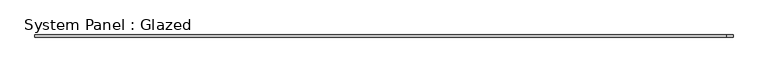
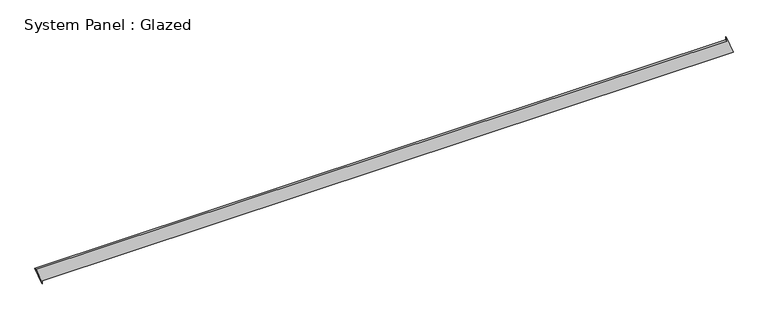
"""IFC4 building model written with IfcOpenShell, lengths in millimetres: plate geometry, System Panel : Glazed."""

from ifc_helpers import new_model, si_unit, frame, origin, place, context, project, spatial, polyline, outline, extrude, source, transform, mapped, element, save


def system_panel_glazed_383bb218(model_context):
    return source(origin(), model_context, "Body", "SweptSolid", [
        extrude(outline(polyline([(0.0, -3956.8326568), (35.3553391, -3956.8326568), (35.3553391, 4027.6791424), (234.6435672, 3956.3630659), (199.2882281, 3956.3621746), (199.4894988, -4027.6791424), (0.0, -3956.8326568)])), frame((0.0, -49.5, 0.0), z_axis=(0.0, 1.0, 0.0), x_axis=(0.0, 0.0, 1.0)), (0.0, 0.0, 1.0), 25.0),
    ])


if __name__ == "__main__":
    model = new_model("IFC4")
    model_context = context("Model", 3, world=origin())
    ifc_project = project(units=[si_unit("LENGTHUNIT", "METRE", prefix="MILLI")], contexts=[model_context])
    site = spatial("IfcSite", under=ifc_project)
    building = spatial("IfcBuilding", under=site)
    placement = place(None, origin())
    system_panel_glazed_shape = system_panel_glazed_383bb218(model_context)
    element("IfcPlate", 1, ObjectType="System Panel : Glazed", at=placement, inside=building, context=model_context, shape_type="MappedRepresentation", body=[
        mapped(system_panel_glazed_shape, transform((0.0, 0.0, 0.0), x_axis=(1.0, 0.0, 0.0), y_axis=(0.0, 1.0, 0.0), z_axis=(0.0, 0.0, 1.0))),
    ])
    save(model, "model.ifc")

# Revit data of these elements
# Element 1 (IfcPlate, "System Panel : Glazed")
#   Materials on its faces: "Glass"
# Materials
#   "Glass": class "Glass", colour RGB 218 227 224, transparency 0.85, Description = "Soda Lime Glass", Cost = 0
